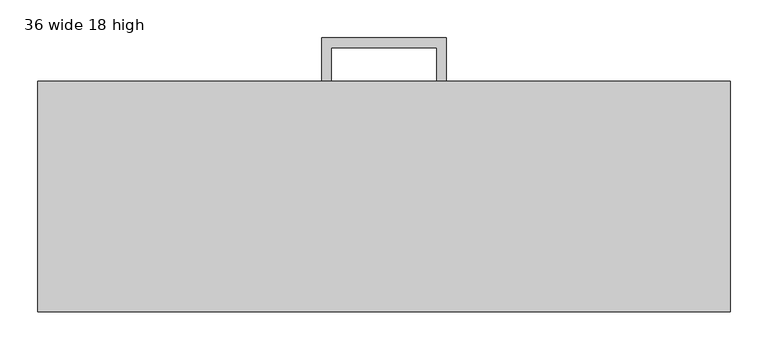
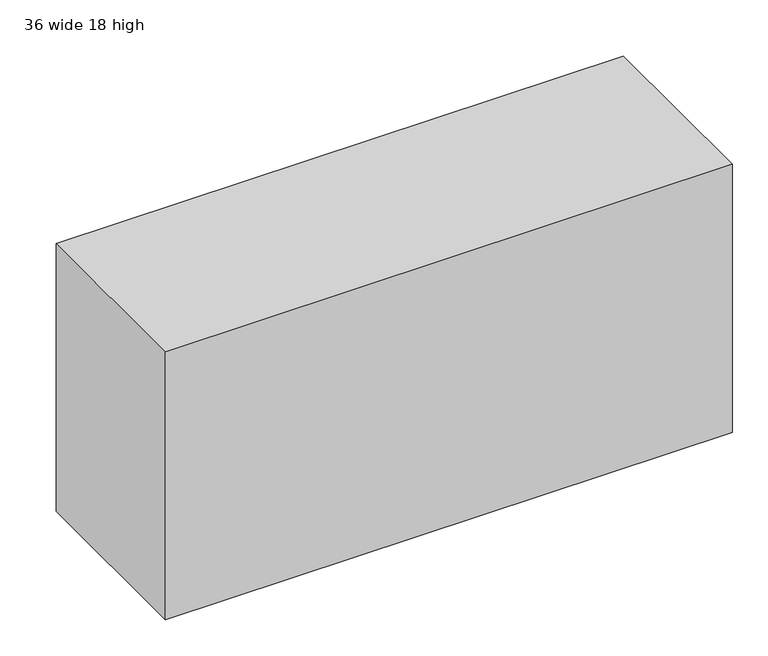
"""IFC4 building model written with IfcOpenShell, lengths in millimetres: furniture geometry, Binder Bin : 36 wide 18 high."""

import ifcopenshell
import ifcopenshell.guid

model = None  # the IFC model being written
_history = None  # IfcOwnerHistory: only IFC2X3 demands one
_inside = {}  # id of a spatial element -> (the spatial element, [elements in it])
_under = {}  # id of a project, library or spatial element -> (it, [spatial elements below it])
_declared = {}  # id of a project -> (the project, [libraries it declares])
_typed = {}  # id of a type object -> (the type object, [elements of that type])
_made_of = {}  # id of a material, layer set ... -> (it, [elements and type objects made of it])


def new_model(schema):
    """Start an empty IFC model of exactly this schema.

    Asked for "IFC4X3", IfcOpenShell would pick the latest addendum, in which some entities
    have other attributes; the version numbers below select the first issue.
    IFC2X3 requires an IfcOwnerHistory on every rooted entity: one is made here for all.
    """
    global model, _history
    if schema == "IFC4X3":
        model = ifcopenshell.file(schema_version=(4, 3, 0, 0))
    else:
        model = ifcopenshell.file(schema=schema)
    _inside.clear()
    _under.clear()
    _declared.clear()
    _typed.clear()
    _made_of.clear()
    _history = None
    if model.schema == "IFC2X3":
        org = make("IfcOrganization", Name="unknown")
        user = make(
            "IfcPersonAndOrganization",
            ThePerson=make("IfcPerson", FamilyName="unknown"),
            TheOrganization=org,
        )
        app = make(
            "IfcApplication",
            ApplicationDeveloper=org,
            Version="unknown",
            ApplicationFullName="unknown",
            ApplicationIdentifier="unknown",
        )
        _history = make(
            "IfcOwnerHistory",
            OwningUser=user,
            OwningApplication=app,
            ChangeAction="ADDED",
            CreationDate=0,
        )
    return model


def make(cls, **values):
    """One entity of the class cls with the attributes given. An attribute that is None is left unset."""
    return model.create_entity(
        cls, **{name: value for name, value in values.items() if value is not None}
    )


def rooted(cls, **values):
    """An entity with a GlobalId (a new one), such as an element, a storey or a relation."""
    return make(cls, GlobalId=ifcopenshell.guid.new(), OwnerHistory=_history, **values)


def si_unit(unit_type, name, prefix=None):
    """IfcSIUnit, for example si_unit("LENGTHUNIT", "METRE", prefix="MILLI")."""
    return make("IfcSIUnit", UnitType=unit_type, Prefix=prefix, Name=name)


def assignment(units):
    """IfcUnitAssignment: the units of a project."""
    return None if units is None else make("IfcUnitAssignment", Units=units)


def point(xyz):
    """IfcCartesianPoint."""
    return None if xyz is None else make("IfcCartesianPoint", Coordinates=xyz)


def direction(xyz):
    """IfcDirection."""
    return None if xyz is None else make("IfcDirection", DirectionRatios=xyz)


def frame(location, z_axis=None, x_axis=None):
    """IfcAxis2Placement3D, a coordinate frame: its origin and axes. An axis left out is left unset."""
    return make(
        "IfcAxis2Placement3D",
        Location=point(location),
        Axis=direction(z_axis),
        RefDirection=direction(x_axis),
    )


def origin():
    """The frame at (0, 0, 0) with its axes left unset."""
    return frame((0.0, 0.0, 0.0))


def place(relative_to, where):
    """IfcLocalPlacement: puts the frame where relative to a parent placement (None: the world)."""
    return make(
        "IfcLocalPlacement", PlacementRelTo=relative_to, RelativePlacement=where
    )


def context(
    kind, dimensions, precision=None, world=None, true_north=None, identifier=None
):
    """IfcGeometricRepresentationContext, for example the 3D "Model" context."""
    return make(
        "IfcGeometricRepresentationContext",
        ContextIdentifier=identifier,
        ContextType=kind,
        CoordinateSpaceDimension=dimensions,
        Precision=precision,
        WorldCoordinateSystem=world,
        TrueNorth=true_north,
    )


def project(units=None, contexts=None):
    """IfcProject with its units and contexts."""
    return rooted(
        "IfcProject",
        Name="project",
        RepresentationContexts=contexts,
        UnitsInContext=assignment(units),
    )


def spatial(cls, under=None, at=None, **own):
    """A site, building, storey or space (cls), placed at a placement, below another one or the project."""
    s = rooted(cls, ObjectPlacement=at, **own)
    if under is not None:
        _under.setdefault(under.id(), (under, []))[1].append(s)
    return s


def polyline(points):
    """IfcPolyline through the points."""
    return make("IfcPolyline", Points=[point(p) for p in points])


def outline(outer, holes=None, kind="AREA"):
    """IfcArbitraryClosedProfileDef: a profile drawn as a closed curve; with holes, ...WithVoids."""
    if holes is None:
        return make("IfcArbitraryClosedProfileDef", ProfileType=kind, OuterCurve=outer)
    return make(
        "IfcArbitraryProfileDefWithVoids",
        ProfileType=kind,
        OuterCurve=outer,
        InnerCurves=holes,
    )


def extrude(swept, where, along, depth):
    """IfcExtrudedAreaSolid: the profile swept, set in the frame where, extruded along a direction by depth."""
    return make(
        "IfcExtrudedAreaSolid",
        SweptArea=swept,
        Position=where,
        ExtrudedDirection=direction(along),
        Depth=depth,
    )


def shape(context_of_items, identifier, shape_type, items):
    """IfcShapeRepresentation: the items that make up one representation, for example the "Body"."""
    return make(
        "IfcShapeRepresentation",
        ContextOfItems=context_of_items,
        RepresentationIdentifier=identifier,
        RepresentationType=shape_type,
        Items=items,
    )


def source(mapping_origin, context_of_items, identifier, shape_type, items):
    """IfcRepresentationMap: a shape defined once, which mapped items show again and again."""
    return make(
        "IfcRepresentationMap",
        MappingOrigin=mapping_origin,
        MappedRepresentation=shape(context_of_items, identifier, shape_type, items),
    )


def transform(
    local_origin,
    x_axis=None,
    y_axis=None,
    z_axis=None,
    scale=None,
    scale2=None,
    scale3=None,
    uniform=True,
):
    """IfcCartesianTransformationOperator3D, or its non-uniform kind. x_axis, y_axis, z_axis: its Axis1, 2, 3."""
    if uniform:
        return make(
            "IfcCartesianTransformationOperator3D",
            Axis1=direction(x_axis),
            Axis2=direction(y_axis),
            LocalOrigin=point(local_origin),
            Scale=scale,
            Axis3=direction(z_axis),
        )
    return make(
        "IfcCartesianTransformationOperator3DnonUniform",
        Axis1=direction(x_axis),
        Axis2=direction(y_axis),
        LocalOrigin=point(local_origin),
        Scale=scale,
        Axis3=direction(z_axis),
        Scale2=scale2,
        Scale3=scale3,
    )


def mapped(mapping_source, mapping_target):
    """IfcMappedItem: shows the shape of a source again, moved by a transform."""
    return make(
        "IfcMappedItem", MappingSource=mapping_source, MappingTarget=mapping_target
    )


def made_of(thing, what):
    """Note that an element or type object is made of a material, layer set ...; save() writes the relation."""
    if what is not None:
        _made_of.setdefault(what.id(), (what, []))[1].append(thing)
    return thing


def element(
    cls,
    number,
    at=None,
    inside=None,
    cuts=None,
    type_object=None,
    material=None,
    context=None,
    identifier="Body",
    shape_type=None,
    held_by="IfcProductDefinitionShape",
    body=None,
    shapes=None,
    **own,
):
    """One element of the class cls, such as IfcWall. Its Tag is "e" and its number.

    at: its placement. inside: the storey or other place that contains it. cuts: it is an
    opening in that element (IfcRelVoidsElement). A single representation is given by context,
    identifier, shape_type and body (its items); several are given by shapes. held_by: the class
    of the entity that holds the representations. save() writes the other relations.
    """
    e = rooted(cls, Tag="e%d" % number, ObjectPlacement=at, **own)
    if body is not None:
        shapes = [shape(context, identifier, shape_type, body)]
    if shapes is not None:
        e.Representation = make(held_by, Representations=shapes)
    if inside is not None:
        _inside.setdefault(inside.id(), (inside, []))[1].append(e)
    if cuts is not None:
        rooted(
            "IfcRelVoidsElement", RelatingBuildingElement=cuts, RelatedOpeningElement=e
        )
    if type_object is not None:
        _typed.setdefault(type_object.id(), (type_object, []))[1].append(e)
    return made_of(e, material)


def aggregate(whole, parts):
    """IfcRelAggregates: a whole, such as a stair, and the parts it consists of."""
    return rooted("IfcRelAggregates", RelatingObject=whole, RelatedObjects=parts)


def save(model, path):
    """Write the relations noted so far, then the file.

    IfcRelAggregates (storeys below a building ...), IfcRelContainedInSpatialStructure (elements
    in a storey), IfcRelDefinesByType, IfcRelAssociatesMaterial and IfcRelDeclares: one each for
    every whole, place, type object, material and project.
    """
    for whole, parts in _under.values():
        aggregate(whole, parts)
    for where, things in _inside.values():
        rooted(
            "IfcRelContainedInSpatialStructure",
            RelatedElements=things,
            RelatingStructure=where,
        )
    for kind, things in _typed.values():
        rooted("IfcRelDefinesByType", RelatedObjects=things, RelatingType=kind)
    for what, things in _made_of.values():
        rooted("IfcRelAssociatesMaterial", RelatedObjects=things, RelatingMaterial=what)
    for by, libraries in _declared.values():
        rooted("IfcRelDeclares", RelatingContext=by, RelatedDefinitions=libraries)
    model.write(path)


def furniture_36_wide_18_high_68bd698f(model_context):
    return source(origin(), model_context, "Body", "SweptSolid", [
        extrude(outline(polyline([(-69.85, 381.0), (-82.55, 381.0), (-82.55, 438.15), (82.55, 438.15), (82.55, 381.0), (69.85, 381.0), (69.85, 425.45), (-69.85, 425.45), (-69.85, 381.0)])), frame((0.0, 0.0, 1568.45), z_axis=(0.0, 0.0, 1.0), x_axis=(1.0, 0.0, 0.0)), (0.0, 0.0, 1.0), 12.7),
        extrude(outline(polyline([(457.2, 76.2), (-457.2, 76.2), (-457.2, 381.0), (457.2, 381.0), (457.2, 76.2)])), frame((0.0, 0.0, 1524.0), z_axis=(0.0, 0.0, 1.0), x_axis=(1.0, 0.0, 0.0)), (0.0, 0.0, 1.0), 457.2),
    ])


if __name__ == "__main__":
    model = new_model("IFC4")
    model_context = context("Model", 3, world=origin())
    ifc_project = project(units=[si_unit("LENGTHUNIT", "METRE", prefix="MILLI")], contexts=[model_context])
    site = spatial("IfcSite", under=ifc_project)
    building = spatial("IfcBuilding", under=site)
    placement = place(None, origin())
    furniture_36_wide_18_high_shape = furniture_36_wide_18_high_68bd698f(model_context)
    element("IfcFurniture", 1, ObjectType="Binder Bin : 36 wide 18 high", at=placement, inside=building, context=model_context, shape_type="MappedRepresentation", body=[
        mapped(furniture_36_wide_18_high_shape, transform((0.0, 0.0, 0.0), x_axis=(1.0, 0.0, 0.0), y_axis=(0.0, 1.0, 0.0), z_axis=(0.0, 0.0, 1.0))),
    ])
    save(model, "model.ifc")

# Revit data of these elements
# Type "Binder Bin : 36 wide 18 high"
#   Width = 3' - 0"
#   Mounting Height [instance default] = 4' - 6"
#   Height = 1' - 6"
#   Default Elevation = 0
# Element 1 (IfcFurniture, "Binder Bin : 36 wide 18 high")
#   Mounting Height = 5' - 0"
